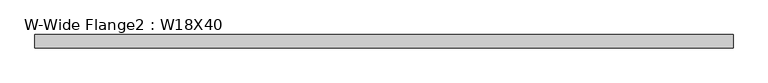
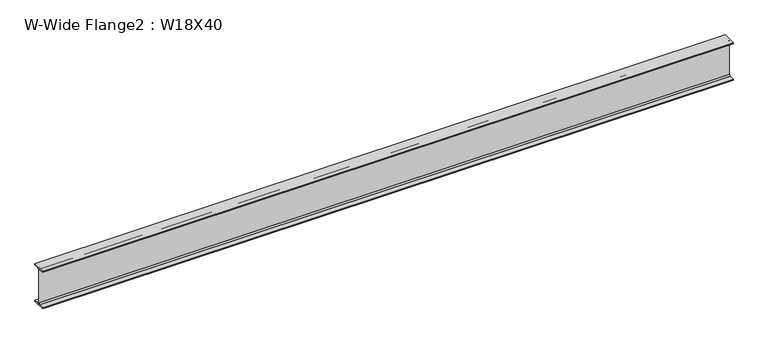
"""IFC4 building model written with IfcOpenShell, lengths in millimetres: beam geometry, W-Wide Flange2 : W18X40."""

from ifc_helpers import new_model, si_unit, point, frame, frame_2d, origin, place, context, project, spatial, polyline, circle_curve, trimmed, segment, composite_curve, outline, extrude, source, transform, mapped, element, save


def w_wide_flange2_w18x40_291d6f15(model_context):
    return source(origin(), model_context, "Body", "SweptSolid", [
        extrude(outline(composite_curve([segment(polyline([(76.454, -213.995), (76.454, -227.33), (-76.454, -227.33), (-76.454, -213.995), (-20.828, -213.995)]), True, "CONTINUOUS"), segment(trimmed(circle_curve(frame_2d((-20.828, -197.1675)), 16.8275), [point((-20.828, -213.995))], [point((-4.0005, -197.1675))], True, "CARTESIAN"), True, "CONTINUOUS"), segment(polyline([(-4.0005, -197.1675), (-4.0005, 197.1675)]), True, "CONTINUOUS"), segment(trimmed(circle_curve(frame_2d((-20.828, 197.1675)), 16.8275), [point((-4.0005, 197.1675))], [point((-20.828, 213.995))], True, "CARTESIAN"), True, "CONTINUOUS"), segment(polyline([(-20.828, 213.995), (-76.454, 213.995), (-76.454, 227.33), (76.454, 227.33), (76.454, 213.995), (20.828, 213.995)]), True, "CONTINUOUS"), segment(trimmed(circle_curve(frame_2d((20.828, 197.1675)), 16.8275), [point((20.828, 213.995))], [point((4.0005, 197.1675))], True, "CARTESIAN"), True, "CONTINUOUS"), segment(polyline([(4.0005, 197.1675), (4.0005, -197.1675)]), True, "CONTINUOUS"), segment(trimmed(circle_curve(frame_2d((20.828, -197.1675)), 16.8275), [point((4.0005, -197.1675))], [point((20.828, -213.995))], True, "CARTESIAN"), True, "CONTINUOUS"), segment(polyline([(20.828, -213.995), (76.454, -213.995)]), True, "CONTINUOUS")], self_intersect=False)), frame((-3917.553125, 0.0, 0.0), z_axis=(1.0, 0.0, 0.0), x_axis=(0.0, 1.0, 0.0)), (0.0, 0.0, 1.0), 7897.415625),
    ])


if __name__ == "__main__":
    model = new_model("IFC4")
    model_context = context("Model", 3, world=origin())
    ifc_project = project(units=[si_unit("LENGTHUNIT", "METRE", prefix="MILLI")], contexts=[model_context])
    site = spatial("IfcSite", under=ifc_project)
    building = spatial("IfcBuilding", under=site)
    placement = place(None, origin())
    w_wide_flange2_w18x40_shape = w_wide_flange2_w18x40_291d6f15(model_context)
    element("IfcBeam", 1, ObjectType="W-Wide Flange2 : W18X40", at=placement, inside=building, context=model_context, shape_type="MappedRepresentation", body=[
        mapped(w_wide_flange2_w18x40_shape, transform((0.0, 0.0, 0.0), x_axis=(1.0, 0.0, 0.0), y_axis=(0.0, 1.0, 0.0), z_axis=(0.0, 0.0, 1.0))),
    ])
    save(model, "model.ifc")

# Revit data of these elements
# Type "W-Wide Flange2 : W18X40"
#   Assembly Code = "B10"
#   W = 40
#   Length [instance default] = 5' - 0"
#   bf = 0' - 6.02"
#   d = 1' - 5.9"
#   k = 0' - 1 3/16"
#   k2 = 0' - 0.6625"
#   tf = 0' - 0.525"
#   tw = 0' - 0.315"
#   A = 0.0819444 SF
#   Structural Material [instance default] = Steel ASTM A992
# Element 1 (IfcBeam, "W-Wide Flange2 : W18X40")
#   Materials on its faces: "Steel ASTM A992"
# Materials
#   "Steel ASTM A992": class "Metal", colour RGB 199 199 199, transparency 0, Description = "Structural steel 50ksi", Cost = 0
